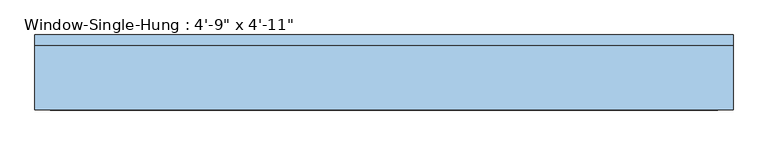
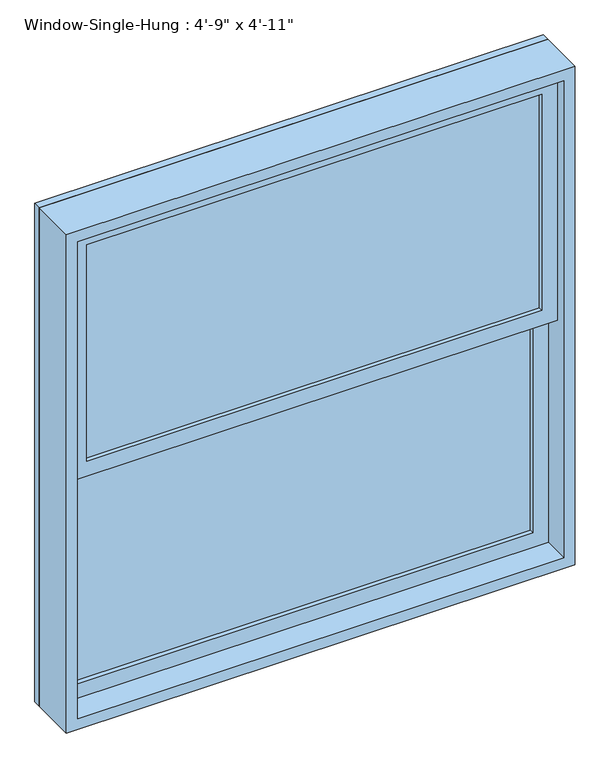
"""IFC4 building model written with IfcOpenShell, lengths in millimetres: window geometry."""

from ifc_helpers import new_model, si_unit, frame, origin, place, context, project, spatial, polyline, outline, extrude, source, transform, mapped, element, save


def window_616431ac(model_context):
    return source(origin(), model_context, "Body", "SweptSolid", [
        extrude(outline(polyline([(647.7, 1.5875), (-647.7, 1.5875), (-647.7, 7.9375), (647.7, 7.9375), (647.7, 1.5875)])), frame((0.0, 0.0, 990.6), z_axis=(0.0, 0.0, 1.0), x_axis=(1.0, 0.0, 0.0)), (0.0, 0.0, 1.0), 650.875),
        extrude(outline(polyline([(-647.7, 14.2875), (-647.7, 20.6375), (647.7, 20.6375), (647.7, 14.2875), (-647.7, 14.2875)])), frame((0.0, 0.0, 990.6), z_axis=(0.0, 0.0, 1.0), x_axis=(1.0, 0.0, 0.0)), (0.0, 0.0, 1.0), 650.875),
        extrude(outline(polyline([(647.7, -42.8625), (-647.7, -42.8625), (-647.7, -36.5125), (647.7, -36.5125), (647.7, -42.8625)])), frame((0.0, 0.0, 1685.925), z_axis=(0.0, 0.0, 1.0), x_axis=(1.0, 0.0, 0.0)), (0.0, 0.0, 1.0), 650.875),
        extrude(outline(polyline([(-647.7, -30.1625), (-647.7, -23.8125), (647.7, -23.8125), (647.7, -30.1625), (-647.7, -30.1625)])), frame((0.0, 0.0, 1685.925), z_axis=(0.0, 0.0, 1.0), x_axis=(1.0, 0.0, 0.0)), (0.0, 0.0, 1.0), 650.875),
        extrude(outline(polyline([(1685.925, 692.15), (1685.925, -692.15), (946.15, -692.15), (946.15, 692.15), (1685.925, 692.15)]), holes=[polyline([(1641.475, -647.7), (1641.475, 647.7), (990.6, 647.7), (990.6, -647.7), (1641.475, -647.7)])]), frame((0.0, -11.1125, 0.0), z_axis=(0.0, 1.0, 0.0), x_axis=(0.0, 0.0, 1.0)), (0.0, 0.0, 1.0), 44.45),
        extrude(outline(polyline([(2381.25, 692.15), (2381.25, -692.15), (1641.475, -692.15), (1641.475, 692.15), (2381.25, 692.15)]), holes=[polyline([(2336.8, -647.7), (2336.8, 647.7), (1685.925, 647.7), (1685.925, -647.7), (2336.8, -647.7)])]), frame((0.0, -55.5625, 0.0), z_axis=(0.0, 1.0, 0.0), x_axis=(0.0, 0.0, 1.0)), (0.0, 0.0, 1.0), 44.45),
        extrude(outline(polyline([(2413.0, 723.9), (2413.0, -723.9), (914.4, -723.9), (914.4, 723.9), (2413.0, 723.9)]), holes=[polyline([(2381.25, -692.15), (2381.25, 692.15), (946.15, 692.15), (946.15, -692.15), (2381.25, -692.15)])]), frame((0.0, -87.3125, 0.0), z_axis=(0.0, 1.0, 0.0), x_axis=(0.0, 0.0, 1.0)), (0.0, 0.0, 1.0), 133.35),
        extrude(outline(polyline([(2413.0, 723.9), (2413.0, -723.9), (914.4, -723.9), (914.4, 723.9), (2413.0, 723.9)]), holes=[polyline([(2393.95, 704.85), (933.45, 704.85), (933.45, -704.85), (2393.95, -704.85), (2393.95, 704.85)])]), frame((0.0, 46.0375, 0.0), z_axis=(0.0, 1.0, 0.0), x_axis=(0.0, 0.0, 1.0)), (0.0, 0.0, 1.0), 22.225),
    ])


if __name__ == "__main__":
    model = new_model("IFC4")
    model_context = context("Model", 3, world=origin())
    ifc_project = project(units=[si_unit("LENGTHUNIT", "METRE", prefix="MILLI")], contexts=[model_context])
    site = spatial("IfcSite", under=ifc_project)
    building = spatial("IfcBuilding", under=site)
    placement = place(None, origin())
    window_shape = window_616431ac(model_context)
    element("IfcWindow", 1, ObjectType="Window-Single-Hung : 4'-9\" x 4'-11\"", at=placement, inside=building, context=model_context, shape_type="MappedRepresentation", body=[
        mapped(window_shape, transform((0.0, 0.0, 0.0), x_axis=(1.0, 0.0, 0.0), y_axis=(0.0, 1.0, 0.0), z_axis=(0.0, 0.0, 1.0))),
    ])
    save(model, "model.ifc")

# Revit data of these elements
# Type "Window-Single-Hung : 4'-9\" x 4'-11\""
#   Type Mark = "23"
#   Fire Rating = "0.5h"
#   Construction Type Id = "DG-DR"
#   Assembly Code = "B2020100"
#   Analytic Construction = "Double glazing - domestic"
#   Wall Thickness [instance default] = 0' - 6"
#   Window Inset [instance default] = 0' - 0"
#   Visual Light Transmittance = 0.81
#   Thermal Resistance (R) = 0.319569 (m²·K)/W
#   Solar Heat Gain Coefficient = 0.76
#   Muntin Width = 4' - 3"
#   Muntin Height = 2' - 1 5/8"
#   Interior Wall Closure [instance default] = 0' - 1 1/2"
#   Rough Width = 4' - 9 1/2"
#   Rough Height = 4' - 11 1/2"
#   Frame Extension [instance default] = 0' - 1 1/4"
#   Exterior Wall Closure [instance default] = 0' - 0 1/2"
#   Extension Jamb [instance default] = 0' - 1 1/2"
#   Heat Transfer Coefficient (U) = 3.12929 W/(m²·K)
#   Height = 4' - 11"
#   Width = 4' - 9"
#   Top Muntin Visibility = yes
#   Indicator Visibility [instance default] = yes
#   Extension Jamb Visibility [instance default] = yes
#   Interior Trim Visibility [instance default] = yes
#   Exterior Trim Visibility [instance default] = yes
#   Bottom Muntin Visibility = yes
#   Muntin Pattern = Muntin Pattern_2x2 : Muntin Pattern_2x2
#   Interior Trim Material = Wood - Stained
#   Interior Trim = Trim-Window-Interior-Flat : Picture Frame
#   Exterior Trim Material = Clad - White
#   Exterior Trim = Trim-Window-Exterior-Flat : with Sill
#   Glass Panel Material = Glass
#   Exterior Frame Material = Clad - White
#   Interior Frame Material = Wood - Stained
#   Wall Closure = (empty or 0)
# Element 1 (IfcWindow, "Window-Single-Hung : 4'-9\" x 4'-11\"")
#   Wall Thickness = 0' - 5 3/8"
#   Extension Jamb = 0' - 0 7/8"
#   Materials on its faces: "Wood - Stained", "Glass", "Clad - White"
# Materials
#   "Wood - Stained": class "Wood", colour RGB 224 178 126, transparency 0, Cost = 0
#   "Clad - White": class "Wood", colour RGB 242 242 238, transparency 0, Cost = 0
#   "Glass": class "Glass", colour RGB 0 128 192, transparency 0.75, Description = "Soda Lime Glass", Cost = 0
